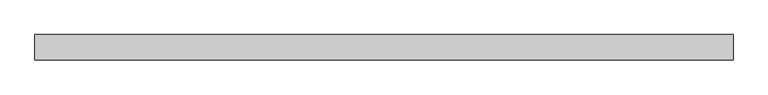
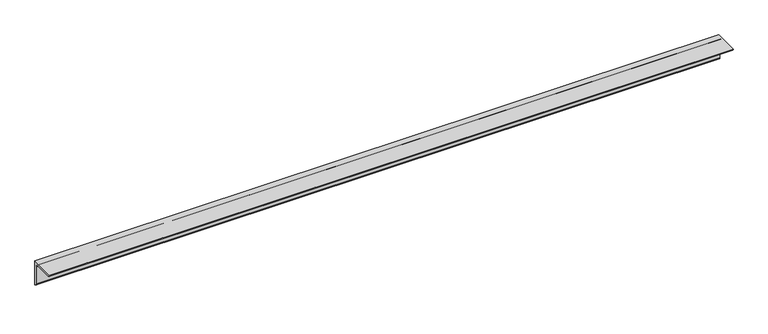
"""IFC4 building model written with IfcOpenShell, lengths in millimetres: member geometry, 0912_Steel Framing_L-KSD3502 : H_SB_AR_S04_L-130x130x12_KBR1."""

from ifc_helpers import new_model, si_unit, point, frame, frame_2d, origin, place, context, project, spatial, polyline, circle_curve, trimmed, segment, composite_curve, outline, extrude, source, transform, mapped, element, save


def member_14297e1c(model_context):
    return source(origin(), model_context, "Body", "SweptSolid", [
        extrude(outline(composite_curve([segment(polyline([(36.4, 36.4), (36.4, -93.6)]), True, "CONTINUOUS"), segment(trimmed(circle_curve(frame_2d((36.4, -81.6)), 12.0), [point((36.4, -93.6))], [point((24.4, -81.6))], False, "CARTESIAN"), True, "CONTINUOUS"), segment(polyline([(24.4, -81.6), (24.4, 12.4)]), True, "CONTINUOUS"), segment(trimmed(circle_curve(frame_2d((12.4, 12.4)), 12.0), [point((24.4, 12.4))], [point((12.4, 24.4))], True, "CARTESIAN"), True, "CONTINUOUS"), segment(polyline([(12.4, 24.4), (-81.6, 24.4)]), True, "CONTINUOUS"), segment(trimmed(circle_curve(frame_2d((-81.6, 36.4)), 12.0), [point((-81.6, 24.4))], [point((-93.6, 36.4))], False, "CARTESIAN"), True, "CONTINUOUS"), segment(polyline([(-93.6, 36.4), (36.4, 36.4)]), True, "CONTINUOUS")], self_intersect=False)), frame((-1819.863551, 0.0, 0.0), z_axis=(1.0, 0.0, 0.0), x_axis=(0.0, 1.0, 0.0)), (0.0, 0.0, 1.0), 3551.9244278),
    ])


if __name__ == "__main__":
    model = new_model("IFC4")
    model_context = context("Model", 3, world=origin())
    ifc_project = project(units=[si_unit("LENGTHUNIT", "METRE", prefix="MILLI")], contexts=[model_context])
    site = spatial("IfcSite", under=ifc_project)
    building = spatial("IfcBuilding", under=site)
    placement = place(None, origin())
    member_shape = member_14297e1c(model_context)
    element("IfcMember", 1, ObjectType="0912_Steel Framing_L-KSD3502 : H_SB_AR_S04_L-130x130x12_KBR1", at=placement, inside=building, context=model_context, shape_type="MappedRepresentation", body=[
        mapped(member_shape, transform((0.0, 0.0, 0.0), x_axis=(1.0, 0.0, 0.0), y_axis=(0.0, 1.0, 0.0), z_axis=(0.0, 0.0, 1.0))),
    ])
    save(model, "model.ifc")

# Revit data of these elements
# Type "0912_Steel Framing_L-KSD3502 : H_SB_AR_S04_L-130x130x12_KBR1"
#   k = 25 mm
#   Perimeter = 0.52 m²/m
#   Nominal Weight = 23.40 kgf/m
#   Length [instance default] = 1000 mm
#   b = 130 mm
#   d = 130 mm
#   t = 12 mm
#   x = 36.4 mm
#   y = 36.4 mm
#   A = 2976.00 m²
#   Structural Material [instance default] = Steel, 45-345
# Element 1 (IfcMember, "0912_Steel Framing_L-KSD3502 : H_SB_AR_S04_L-130x130x12_KBR1")
#   Materials on its faces: "Steel, 45-345"
# Materials
#   "Steel, 45-345": class "Metal", colour RGB 189 187 185, transparency 0, Description = "Steel 345 MPa", Cost = 0
